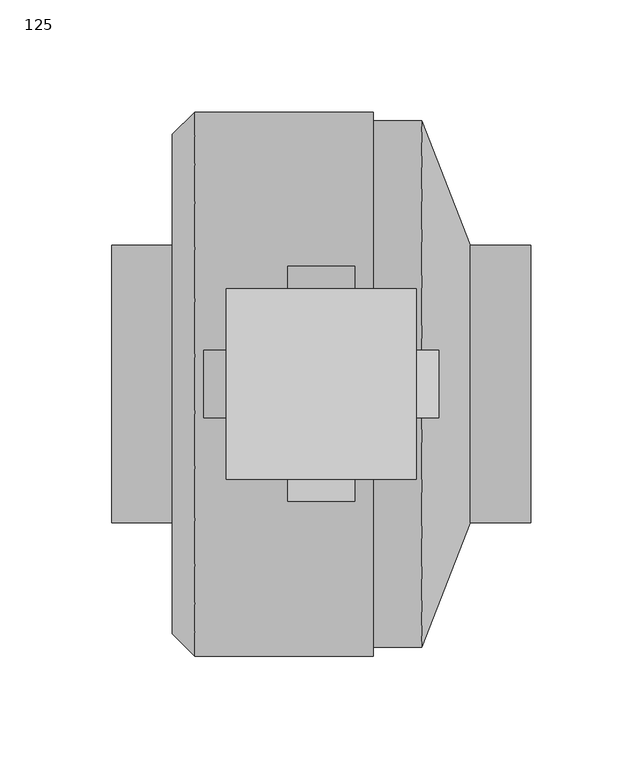
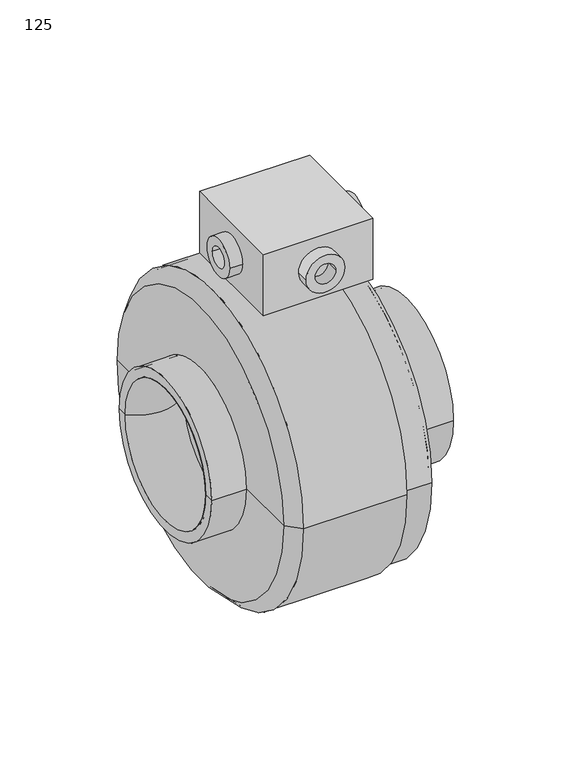
"""IFC4 building model written with IfcOpenShell, lengths in millimetres: proxy geometry, ВЕЗА_Канал-ВЕНТ : 125."""

from ifc_helpers import new_model, si_unit, point, frame, frame_2d, origin, place, context, project, spatial, polyline, circle_curve, ellipse_curve, trimmed, segment, composite_curve, outline, extrude, source, transform, mapped, element, save
from ifc_brep_helpers import plane_surface, cylinder_surface, revolved_surface, advanced_brep


def proxy_125_3bba99a2(model_context):
    return source(origin(), model_context, "Body", "SolidModel", [
        extrude(outline(composite_curve([segment(trimmed(circle_curve(frame_2d((0.0, 147.0)), 15.0), [point((-15.0, 147.0))], [point((15.0, 147.0))], False, "CARTESIAN"), True, "CONTINUOUS"), segment(trimmed(circle_curve(frame_2d((0.0, 147.0)), 15.0), [point((15.0, 147.0))], [point((-15.0, 147.0))], False, "CARTESIAN"), True, "CONTINUOUS")], self_intersect=False), holes=[composite_curve([segment(trimmed(circle_curve(frame_2d((0.0, 147.0)), 8.0), [point((-8.0, 147.0))], [point((8.0, 147.0))], True, "CARTESIAN"), True, "CONTINUOUS"), segment(trimmed(circle_curve(frame_2d((0.0, 147.0)), 8.0), [point((8.0, 147.0))], [point((-8.0, 147.0))], True, "CARTESIAN"), True, "CONTINUOUS")], self_intersect=False)]), frame((42.5, 0.0, 0.0), z_axis=(1.0, 0.0, 0.0), x_axis=(0.0, 1.0, 0.0)), (0.0, 0.0, 1.0), 10.0),
        extrude(outline(composite_curve([segment(trimmed(circle_curve(frame_2d((0.0, 147.0)), 15.0), [point((-15.0, 147.0))], [point((15.0, 147.0))], False, "CARTESIAN"), True, "CONTINUOUS"), segment(trimmed(circle_curve(frame_2d((0.0, 147.0)), 15.0), [point((15.0, 147.0))], [point((-15.0, 147.0))], False, "CARTESIAN"), True, "CONTINUOUS")], self_intersect=False), holes=[composite_curve([segment(trimmed(circle_curve(frame_2d((0.0, 147.0)), 8.0), [point((-8.0, 147.0))], [point((8.0, 147.0))], True, "CARTESIAN"), True, "CONTINUOUS"), segment(trimmed(circle_curve(frame_2d((0.0, 147.0)), 8.0), [point((8.0, 147.0))], [point((-8.0, 147.0))], True, "CARTESIAN"), True, "CONTINUOUS")], self_intersect=False)]), frame((-52.5, 0.0, 0.0), z_axis=(1.0, 0.0, 0.0), x_axis=(0.0, 1.0, 0.0)), (0.0, 0.0, 1.0), 10.0),
        extrude(outline(composite_curve([segment(trimmed(circle_curve(frame_2d((147.0, 0.0)), 15.0), [point((147.0, 15.0))], [point((147.0, -15.0))], False, "CARTESIAN"), True, "CONTINUOUS"), segment(trimmed(circle_curve(frame_2d((147.0, 0.0)), 15.0), [point((147.0, -15.0))], [point((147.0, 15.0))], False, "CARTESIAN"), True, "CONTINUOUS")], self_intersect=False), holes=[composite_curve([segment(trimmed(circle_curve(frame_2d((147.0, 0.0)), 8.0), [point((147.0, 8.0))], [point((147.0, -8.0))], True, "CARTESIAN"), True, "CONTINUOUS"), segment(trimmed(circle_curve(frame_2d((147.0, 0.0)), 8.0), [point((147.0, -8.0))], [point((147.0, 8.0))], True, "CARTESIAN"), True, "CONTINUOUS")], self_intersect=False)]), frame((0.0, -52.5, 0.0), z_axis=(0.0, 1.0, 0.0), x_axis=(0.0, 0.0, 1.0)), (0.0, 0.0, 1.0), 10.0),
        extrude(outline(composite_curve([segment(trimmed(circle_curve(frame_2d((147.0, 0.0)), 15.0), [point((147.0, 15.0))], [point((147.0, -15.0))], False, "CARTESIAN"), True, "CONTINUOUS"), segment(trimmed(circle_curve(frame_2d((147.0, 0.0)), 15.0), [point((147.0, -15.0))], [point((147.0, 15.0))], False, "CARTESIAN"), True, "CONTINUOUS")], self_intersect=False), holes=[composite_curve([segment(trimmed(circle_curve(frame_2d((147.0, 0.0)), 8.0), [point((147.0, 8.0))], [point((147.0, -8.0))], True, "CARTESIAN"), True, "CONTINUOUS"), segment(trimmed(circle_curve(frame_2d((147.0, 0.0)), 8.0), [point((147.0, -8.0))], [point((147.0, 8.0))], True, "CARTESIAN"), True, "CONTINUOUS")], self_intersect=False)]), frame((0.0, 42.5, 0.0), z_axis=(0.0, 1.0, 0.0), x_axis=(0.0, 0.0, 1.0)), (0.0, 0.0, 1.0), 10.0),
        extrude(outline(polyline([(-42.5, -42.5), (-42.5, 42.5), (42.5, 42.5), (42.5, -42.5), (-42.5, -42.5)])), frame((0.0, 0.0, 121.5), z_axis=(0.0, 0.0, 1.0), x_axis=(1.0, 0.0, 0.0)), (0.0, 0.0, 1.0), 50.0),
        advanced_brep(
        [(-93.5, -54.0, 0.0), (-93.5, 54.0, 0.0), (-92.0, 54.0, 0.0), (-92.0, -54.0, 0.0), (-48.5, -54.0, 0.0), (-48.5, 54.0, 0.0), (-50.0, -54.0, 0.0), (-50.0, 54.0, 0.0)],
        [
            (0, 1, circle_curve(frame((-93.5, 0.0, 0.0), z_axis=(1.0, 0.0, 0.0), x_axis=(0.0, 1.0, 0.0)), 54.0)),
            (1, 2),
            (2, 3, circle_curve(frame((-92.0, 0.0, 0.0), z_axis=(-1.0, 0.0, 0.0), x_axis=(0.0, 1.0, 0.0)), 54.0)),
            (3, 0),
            (1, 0, circle_curve(frame((-93.5, 0.0, 0.0), z_axis=(1.0, 0.0, 0.0), x_axis=(0.0, 1.0, 0.0)), 54.0)),
            (3, 2, circle_curve(frame((-92.0, 0.0, 0.0), z_axis=(-1.0, 0.0, 0.0), x_axis=(0.0, 1.0, 0.0)), 54.0)),
            (4, 5, circle_curve(frame((-48.5, 0.0, 0.0), z_axis=(1.0, 0.0, 0.0), x_axis=(0.0, 1.0, 0.0)), 54.0)),
            (5, 1, circle_curve(frame((-71.0, 77.6335583, 0.0), z_axis=(0.0, 0.0, -1.0), x_axis=(1.0, 0.0, 0.0)), 32.6311979)),
            (0, 4, circle_curve(frame((-71.0, -77.6335583, 0.0), z_axis=(0.0, 0.0, -1.0), x_axis=(1.0, 0.0, 0.0)), 32.6311979)),
            (5, 4, circle_curve(frame((-48.5, 0.0, 0.0), z_axis=(1.0, 0.0, 0.0), x_axis=(0.0, 1.0, 0.0)), 54.0)),
            (6, 7, circle_curve(frame((-50.0, 0.0, 0.0), z_axis=(1.0, 0.0, 0.0), x_axis=(0.0, 1.0, 0.0)), 54.0)),
            (7, 5),
            (4, 6),
            (7, 6, circle_curve(frame((-50.0, 0.0, 0.0), z_axis=(1.0, 0.0, 0.0), x_axis=(0.0, 1.0, 0.0)), 54.0)),
            (2, 7, circle_curve(frame((-71.0, 77.7023679, 0.0), z_axis=(0.0, 0.0, 1.0), x_axis=(1.0, 0.0, 0.0)), 31.667053)),
            (6, 3, circle_curve(frame((-71.0, -77.7023679, 0.0), z_axis=(0.0, 0.0, 1.0), x_axis=(1.0, 0.0, 0.0)), 31.667053)),
        ],
        [
            cylinder_surface(frame((-138.5, 0.0, 0.0), z_axis=(-1.0, 0.0, 0.0), x_axis=(0.0, 1.0, 0.0)), 54.0),
            revolved_surface(trimmed(ellipse_curve(frame((-71.0, 77.6335583, 0.0), z_axis=(0.0, 0.0, 1.0), x_axis=(1.0, 0.0, 0.0)), 32.6311979, 32.6311979), [point((-93.5, 54.0, 0.0))], [point((-48.5, 54.0, 0.0))], True, "CARTESIAN"), (-138.5, 0.0, 0.0), (-1.0, 0.0, 0.0)),
            revolved_surface(trimmed(ellipse_curve(frame((-71.0, 77.7023679, 0.0), z_axis=(0.0, 0.0, -1.0), x_axis=(1.0, 0.0, 0.0)), 31.667053, 31.667053), [point((-50.0, 54.0, 0.0))], [point((-92.0, 54.0, 0.0))], True, "CARTESIAN"), (-138.5, 0.0, 0.0), (-1.0, 0.0, 0.0)),
        ],
        [
            (0, [[1, 2, 3, 4]]),
            (0, [[5, -4, 6, -2]]),
            (1, [[7, 8, -1, 9]]),
            (1, [[10, -9, -5, -8]]),
            (0, [[11, 12, -7, 13]]),
            (0, [[14, -13, -10, -12]]),
            (2, [[-3, 15, -11, 16]]),
            (2, [[-6, -16, -14, -15]]),
        ],
    ),
        advanced_brep(
        [(-92.0, -60.5, 0.0), (-92.0, 60.5, 0.0), (-92.0, 54.0, 0.0), (-92.0, -54.0, 0.0), (21.6666667, -120.0, 0.0), (21.6666667, 120.0, 0.0), (-56.5, 120.0, 0.0), (-56.5, -120.0, 0.0), (21.6666667, -116.0, 0.0), (21.6666667, 116.0, 0.0), (43.3333333, -116.0, 0.0), (43.3333333, 116.0, 0.0), (65.0, -60.5, 0.0), (65.0, 60.5, 0.0), (93.5, -60.5, 0.0), (93.5, 60.5, 0.0), (93.5, -62.0, 0.0), (93.5, 62.0, 0.0), (66.5, -62.0, 0.0), (66.5, 62.0, 0.0), (44.8333333, -117.5, 0.0), (44.8333333, 117.5, 0.0), (23.1666667, -117.5, 0.0), (23.1666667, 117.5, 0.0), (23.1666667, -121.5, 0.0), (23.1666667, 121.5, 0.0), (-56.5, -121.5, 0.0), (-56.5, 121.5, 0.0), (-66.5, -62.0, 0.0), (-66.5, 62.0, 0.0), (-66.5, 111.5, 0.0), (-66.5, -111.5, 0.0), (-93.5, -62.0, 0.0), (-93.5, 62.0, 0.0), (-93.5, -54.0, 0.0), (-93.5, 54.0, 0.0), (-65.0, -60.5, 0.0), (-65.0, 60.5, 0.0), (-65.0, -111.5, 0.0), (-65.0, 111.5, 0.0)],
        [
            (0, 1, circle_curve(frame((-92.0, 0.0, 0.0), z_axis=(1.0, 0.0, 0.0), x_axis=(0.0, 1.0, 0.0)), 60.5)),
            (1, 2),
            (2, 3, circle_curve(frame((-92.0, 0.0, 0.0), z_axis=(-1.0, 0.0, 0.0), x_axis=(0.0, 1.0, 0.0)), 54.0)),
            (3, 0),
            (1, 0, circle_curve(frame((-92.0, 0.0, 0.0), z_axis=(1.0, 0.0, 0.0), x_axis=(0.0, 1.0, 0.0)), 60.5)),
            (3, 2, circle_curve(frame((-92.0, 0.0, 0.0), z_axis=(-1.0, 0.0, 0.0), x_axis=(0.0, 1.0, 0.0)), 54.0)),
            (4, 5, circle_curve(frame((21.6666667, 0.0, 0.0), z_axis=(1.0, 0.0, 0.0), x_axis=(0.0, 1.0, 0.0)), 120.0)),
            (5, 6),
            (6, 7, circle_curve(frame((-56.5, 0.0, 0.0), z_axis=(-1.0, 0.0, 0.0), x_axis=(0.0, 1.0, 0.0)), 120.0)),
            (7, 4),
            (5, 4, circle_curve(frame((21.6666667, 0.0, 0.0), z_axis=(1.0, 0.0, 0.0), x_axis=(0.0, 1.0, 0.0)), 120.0)),
            (7, 6, circle_curve(frame((-56.5, 0.0, 0.0), z_axis=(-1.0, 0.0, 0.0), x_axis=(0.0, 1.0, 0.0)), 120.0)),
            (8, 9, circle_curve(frame((21.6666667, 0.0, 0.0), z_axis=(1.0, 0.0, 0.0), x_axis=(0.0, 1.0, 0.0)), 116.0)),
            (9, 5),
            (4, 8),
            (9, 8, circle_curve(frame((21.6666667, 0.0, 0.0), z_axis=(1.0, 0.0, 0.0), x_axis=(0.0, 1.0, 0.0)), 116.0)),
            (10, 11, circle_curve(frame((43.3333333, 0.0, 0.0), z_axis=(1.0, 0.0, 0.0), x_axis=(0.0, 1.0, 0.0)), 116.0)),
            (11, 9),
            (8, 10),
            (11, 10, circle_curve(frame((43.3333333, 0.0, 0.0), z_axis=(1.0, 0.0, 0.0), x_axis=(0.0, 1.0, 0.0)), 116.0)),
            (12, 13, circle_curve(frame((65.0, 0.0, 0.0), z_axis=(1.0, 0.0, 0.0), x_axis=(0.0, 1.0, 0.0)), 60.5)),
            (13, 11),
            (10, 12),
            (13, 12, circle_curve(frame((65.0, 0.0, 0.0), z_axis=(1.0, 0.0, 0.0), x_axis=(0.0, 1.0, 0.0)), 60.5)),
            (14, 15, circle_curve(frame((93.5, 0.0, 0.0), z_axis=(1.0, 0.0, 0.0), x_axis=(0.0, 1.0, 0.0)), 60.5)),
            (15, 13),
            (12, 14),
            (15, 14, circle_curve(frame((93.5, 0.0, 0.0), z_axis=(1.0, 0.0, 0.0), x_axis=(0.0, 1.0, 0.0)), 60.5)),
            (16, 17, circle_curve(frame((93.5, 0.0, 0.0), z_axis=(1.0, 0.0, 0.0), x_axis=(0.0, 1.0, 0.0)), 62.0)),
            (17, 15),
            (14, 16),
            (17, 16, circle_curve(frame((93.5, 0.0, 0.0), z_axis=(1.0, 0.0, 0.0), x_axis=(0.0, 1.0, 0.0)), 62.0)),
            (18, 19, circle_curve(frame((66.5, 0.0, 0.0), z_axis=(1.0, 0.0, 0.0), x_axis=(0.0, 1.0, 0.0)), 62.0)),
            (19, 17),
            (16, 18),
            (19, 18, circle_curve(frame((66.5, 0.0, 0.0), z_axis=(1.0, 0.0, 0.0), x_axis=(0.0, 1.0, 0.0)), 62.0)),
            (20, 21, circle_curve(frame((44.8333333, 0.0, 0.0), z_axis=(1.0, 0.0, 0.0), x_axis=(0.0, 1.0, 0.0)), 117.5)),
            (21, 19),
            (18, 20),
            (21, 20, circle_curve(frame((44.8333333, 0.0, 0.0), z_axis=(1.0, 0.0, 0.0), x_axis=(0.0, 1.0, 0.0)), 117.5)),
            (22, 23, circle_curve(frame((23.1666667, 0.0, 0.0), z_axis=(1.0, 0.0, 0.0), x_axis=(0.0, 1.0, 0.0)), 117.5)),
            (23, 21),
            (20, 22),
            (23, 22, circle_curve(frame((23.1666667, 0.0, 0.0), z_axis=(1.0, 0.0, 0.0), x_axis=(0.0, 1.0, 0.0)), 117.5)),
            (24, 25, circle_curve(frame((23.1666667, 0.0, 0.0), z_axis=(1.0, 0.0, 0.0), x_axis=(0.0, 1.0, 0.0)), 121.5)),
            (25, 23),
            (22, 24),
            (25, 24, circle_curve(frame((23.1666667, 0.0, 0.0), z_axis=(1.0, 0.0, 0.0), x_axis=(0.0, 1.0, 0.0)), 121.5)),
            (26, 27, circle_curve(frame((-56.5, 0.0, 0.0), z_axis=(1.0, 0.0, 0.0), x_axis=(0.0, 1.0, 0.0)), 121.5)),
            (27, 25),
            (24, 26),
            (27, 26, circle_curve(frame((-56.5, 0.0, 0.0), z_axis=(1.0, 0.0, 0.0), x_axis=(0.0, 1.0, 0.0)), 121.5)),
            (28, 29, circle_curve(frame((-66.5, 0.0, 0.0), z_axis=(1.0, 0.0, 0.0), x_axis=(0.0, 1.0, 0.0)), 62.0)),
            (29, 30),
            (30, 31, circle_curve(frame((-66.5, 0.0, 0.0), z_axis=(-1.0, 0.0, 0.0), x_axis=(0.0, 1.0, 0.0)), 111.5)),
            (31, 28),
            (29, 28, circle_curve(frame((-66.5, 0.0, 0.0), z_axis=(1.0, 0.0, 0.0), x_axis=(0.0, 1.0, 0.0)), 62.0)),
            (31, 30, circle_curve(frame((-66.5, 0.0, 0.0), z_axis=(-1.0, 0.0, 0.0), x_axis=(0.0, 1.0, 0.0)), 111.5)),
            (32, 33, circle_curve(frame((-93.5, 0.0, 0.0), z_axis=(1.0, 0.0, 0.0), x_axis=(0.0, 1.0, 0.0)), 62.0)),
            (33, 29),
            (28, 32),
            (33, 32, circle_curve(frame((-93.5, 0.0, 0.0), z_axis=(1.0, 0.0, 0.0), x_axis=(0.0, 1.0, 0.0)), 62.0)),
            (34, 35, circle_curve(frame((-93.5, 0.0, 0.0), z_axis=(1.0, 0.0, 0.0), x_axis=(0.0, 1.0, 0.0)), 54.0)),
            (35, 33),
            (32, 34),
            (35, 34, circle_curve(frame((-93.5, 0.0, 0.0), z_axis=(1.0, 0.0, 0.0), x_axis=(0.0, 1.0, 0.0)), 54.0)),
            (2, 35),
            (34, 3),
            (36, 37, circle_curve(frame((-65.0, 0.0, 0.0), z_axis=(1.0, 0.0, 0.0), x_axis=(0.0, 1.0, 0.0)), 60.5)),
            (37, 1),
            (0, 36),
            (37, 36, circle_curve(frame((-65.0, 0.0, 0.0), z_axis=(1.0, 0.0, 0.0), x_axis=(0.0, 1.0, 0.0)), 60.5)),
            (38, 39, circle_curve(frame((-65.0, 0.0, 0.0), z_axis=(1.0, 0.0, 0.0), x_axis=(0.0, 1.0, 0.0)), 111.5)),
            (39, 37),
            (36, 38),
            (39, 38, circle_curve(frame((-65.0, 0.0, 0.0), z_axis=(1.0, 0.0, 0.0), x_axis=(0.0, 1.0, 0.0)), 111.5)),
            (6, 39),
            (38, 7),
            (30, 27),
            (26, 31),
        ],
        [
            plane_surface(frame((-92.0, 0.0, 0.0), z_axis=(1.0, 0.0, 0.0), x_axis=(0.0, 1.0, 0.0))),
            revolved_surface(polyline([(-56.5, 120.0, 0.0), (21.666666700000007, 120.0, 0.0)]), (-163.5, 0.0, 0.0), (-1.0, 0.0, 0.0)),
            plane_surface(frame((21.6666667, 0.0, 0.0), z_axis=(-1.0, 0.0, 0.0), x_axis=(0.0, 1.0, 0.0))),
            revolved_surface(polyline([(21.666666700000007, 116.0, 0.0), (43.33333329999999, 116.0, 0.0)]), (-163.5, 0.0, 0.0), (-1.0, 0.0, 0.0)),
            revolved_surface(polyline([(43.3333333, 116.0, 0.0), (65.0, 60.5, 0.0)]), (-163.5, 0.0, 0.0), (-1.0, 0.0, 0.0)),
            revolved_surface(polyline([(65.0, 60.5, 0.0), (93.5, 60.5, 0.0)]), (-163.5, 0.0, 0.0), (-1.0, 0.0, 0.0)),
            plane_surface(frame((93.5, 0.0, 0.0), z_axis=(1.0, 0.0, 0.0), x_axis=(0.0, 1.0, 0.0))),
            cylinder_surface(frame((-163.5, 0.0, 0.0), z_axis=(-1.0, 0.0, 0.0), x_axis=(0.0, 1.0, 0.0)), 62.0),
            revolved_surface(polyline([(66.5, 62.0, 0.0), (44.8333333, 117.5, 0.0)]), (-163.5, 0.0, 0.0), (-1.0, 0.0, 0.0)),
            cylinder_surface(frame((-163.5, 0.0, 0.0), z_axis=(-1.0, 0.0, 0.0), x_axis=(0.0, 1.0, 0.0)), 117.5),
            plane_surface(frame((23.1666667, 0.0, 0.0), z_axis=(1.0, 0.0, 0.0), x_axis=(0.0, 1.0, 0.0))),
            cylinder_surface(frame((-163.5, 0.0, 0.0), z_axis=(-1.0, 0.0, 0.0), x_axis=(0.0, 1.0, 0.0)), 121.5),
            plane_surface(frame((-66.5, 0.0, 0.0), z_axis=(-1.0, 0.0, 0.0), x_axis=(0.0, 1.0, 0.0))),
            plane_surface(frame((-93.5, 0.0, 0.0), z_axis=(-1.0, 0.0, 0.0), x_axis=(0.0, 1.0, 0.0))),
            revolved_surface(polyline([(-93.5, 54.0, 0.0), (-92.0, 54.0, 0.0)]), (-163.5, 0.0, 0.0), (-1.0, 0.0, 0.0)),
            revolved_surface(polyline([(-92.0, 60.5, 0.0), (-65.0, 60.5, 0.0)]), (-163.5, 0.0, 0.0), (-1.0, 0.0, 0.0)),
            plane_surface(frame((-65.0, 0.0, 0.0), z_axis=(1.0, 0.0, 0.0), x_axis=(0.0, 1.0, 0.0))),
            revolved_surface(polyline([(-65.0, 111.5, 0.0), (-56.5, 120.0, 0.0)]), (-163.5, 0.0, 0.0), (-1.0, 0.0, 0.0)),
            revolved_surface(polyline([(-56.5, 121.5, 0.0), (-66.5, 111.5, 0.0)]), (-163.5, 0.0, 0.0), (-1.0, 0.0, 0.0)),
        ],
        [
            (0, [[1, 2, 3, 4]]),
            (0, [[5, -4, 6, -2]]),
            (1, [[7, 8, 9, 10]]),
            (1, [[11, -10, 12, -8]]),
            (2, [[13, 14, -7, 15]]),
            (2, [[16, -15, -11, -14]]),
            (3, [[17, 18, -13, 19]]),
            (3, [[20, -19, -16, -18]]),
            (4, [[21, 22, -17, 23]]),
            (4, [[24, -23, -20, -22]]),
            (5, [[25, 26, -21, 27]]),
            (5, [[28, -27, -24, -26]]),
            (6, [[29, 30, -25, 31]]),
            (6, [[32, -31, -28, -30]]),
            (7, [[33, 34, -29, 35]]),
            (7, [[36, -35, -32, -34]]),
            (8, [[37, 38, -33, 39]]),
            (8, [[40, -39, -36, -38]]),
            (9, [[41, 42, -37, 43]]),
            (9, [[44, -43, -40, -42]]),
            (10, [[45, 46, -41, 47]]),
            (10, [[48, -47, -44, -46]]),
            (11, [[49, 50, -45, 51]]),
            (11, [[52, -51, -48, -50]]),
            (12, [[53, 54, 55, 56]]),
            (12, [[57, -56, 58, -54]]),
            (7, [[59, 60, -53, 61]]),
            (7, [[62, -61, -57, -60]]),
            (13, [[63, 64, -59, 65]]),
            (13, [[66, -65, -62, -64]]),
            (14, [[-3, 67, -63, 68]]),
            (14, [[-6, -68, -66, -67]]),
            (15, [[69, 70, -1, 71]]),
            (15, [[72, -71, -5, -70]]),
            (16, [[73, 74, -69, 75]]),
            (16, [[76, -75, -72, -74]]),
            (17, [[-9, 77, -73, 78]]),
            (17, [[-12, -78, -76, -77]]),
            (18, [[-55, 79, -49, 80]]),
            (18, [[-58, -80, -52, -79]]),
        ],
    ),
        advanced_brep(
        [(0.0, -91.75, 0.0), (0.0, 91.75, 0.0), (0.0, 0.0, 0.0), (-48.5, -91.75, 0.0), (-48.5, 91.75, 0.0), (-48.5, 0.0, 0.0)],
        [
            (0, 1, circle_curve(frame((0.0, 0.0, 0.0), z_axis=(1.0, 0.0, 0.0), x_axis=(0.0, 1.0, 0.0)), 91.75)),
            (1, 2),
            (2, 0),
            (1, 0, circle_curve(frame((0.0, 0.0, 0.0), z_axis=(1.0, 0.0, 0.0), x_axis=(0.0, 1.0, 0.0)), 91.75)),
            (3, 4, circle_curve(frame((-48.5, 0.0, 0.0), z_axis=(1.0, 0.0, 0.0), x_axis=(0.0, 1.0, 0.0)), 91.75)),
            (4, 1),
            (0, 3),
            (4, 3, circle_curve(frame((-48.5, 0.0, 0.0), z_axis=(1.0, 0.0, 0.0), x_axis=(0.0, 1.0, 0.0)), 91.75)),
            (5, 4),
            (3, 5),
        ],
        [
            plane_surface(frame((0.0, 0.0, 0.0), z_axis=(1.0, 0.0, 0.0), x_axis=(0.0, 1.0, 0.0))),
            cylinder_surface(frame((-183.5, 0.0, 0.0), z_axis=(-1.0, 0.0, 0.0), x_axis=(0.0, 1.0, 0.0)), 91.75),
            plane_surface(frame((-48.5, 0.0, 0.0), z_axis=(-1.0, 0.0, 0.0), x_axis=(0.0, 1.0, 0.0))),
        ],
        [
            (0, [[1, 2, 3]]),
            (0, [[4, -3, -2]]),
            (1, [[5, 6, -1, 7]]),
            (1, [[8, -7, -4, -6]]),
            (2, [[9, -5, 10]]),
            (2, [[-10, -8, -9]]),
        ],
    ),
    ])


if __name__ == "__main__":
    model = new_model("IFC4")
    model_context = context("Model", 3, world=origin())
    ifc_project = project(units=[si_unit("LENGTHUNIT", "METRE", prefix="MILLI")], contexts=[model_context])
    site = spatial("IfcSite", under=ifc_project)
    building = spatial("IfcBuilding", under=site)
    placement = place(None, origin())
    proxy_125_shape = proxy_125_3bba99a2(model_context)
    element("IfcBuildingElementProxy", 1, Name="ВЕЗА_Канал-ВЕНТ : 125", ObjectType="ВЕЗА_Канал-ВЕНТ : 125", at=placement, inside=building, context=model_context, shape_type="MappedRepresentation", body=[
        mapped(proxy_125_shape, transform((0.0, 0.0, 0.0), x_axis=(1.0, 0.0, 0.0), y_axis=(0.0, 1.0, 0.0), z_axis=(0.0, 0.0, 1.0))),
    ])
    save(model, "model.ifc")

# Revit data of these elements
# Type "ВЕЗА_Канал-ВЕНТ : 125"
#   ВЕЗА_Классификатор = "11031"
#   ВЕЗА_Контакты = "bim@veza.ru"
#   URL = "http://www.veza.ru/docs/sistemy-kanalnoy-ventilyatsii-kanal/"
#   Таблица = "kanal-vent"
#   ADSK_Примечание = ""
#   ADSK_Позиция на схеме = ""
#   ADSK_Позиция = ""
#   ADSK_Наименование краткое = "Канал-ВЕНТ"
#   ADSK_Наименование = "Вентилятор канальный для круглых каналов"
#   ADSK_Марка = "Канал-ВЕНТ-125"
#   ADSK_Комплект [instance default] = ""
#   ADSK_Код изделия = ""
#   ADSK_Завод-изготовитель = "ООО \"Веза\", Россия, Москва, ИНН 505001001, info@veza.ru"
#   ADSK_Единица измерения = "компл."
#   ADSK_Дата изменения = "10.03.2020"
#   ADSK_Группирование = ""
#   ADSK_Версия семейства = "Версия 4"
#   ADSK_Версия Revit = "Revit 2017"
#   Угол поворота УГО 3D [instance default] = 45°
#   L [instance default] = 187 mm
#   h [instance default] = 27 mm
#   D [instance default] = 243 mm
#   ADSK_Ток [instance default] = 0.29 A
#   ADSK_Расход воздуха [instance default] = 561.6 m³/h
#   ADSK_Размер_Диаметр [instance default] = 124 mm
#   ADSK_Полная мощность [instance default] = 65 VA
#   ADSK_Номинальная мощность [instance default] = 65 W
#   ADSK_Напряжение = 230 V
#   ADSK_Масса [instance default] = 3.3
#   ADSK_Коэффициент мощности = 1
#   ADSK_Количество = 1
#   Масштаб УГО [instance default] = 100
#   ВЕЗА_Типоразмер = 125
#   ВЕЗА_Число полюсов = 2
#   ADSK_Частота вращения двигателя [instance default] = 2400
#   ADSK_Количество фаз = 1
#   Материал = ВЕЗА_Оцинкованная сталь
#   Default Elevation = 0
#   Description = (empty or 0)
#   Type Image = (empty or 0)
#   Manufacturer = ""
# Element 1 (IfcBuildingElementProxy, "ВЕЗА_Канал-ВЕНТ : 125")
#   Materials on its faces: "ВЕЗА_Оцинкованная сталь", "Пластмасса коробки"
# Materials
#   "ВЕЗА_Оцинкованная сталь": class "Типовые", colour RGB 120 120 120, transparency 0, Cost = 0
#   "Пластмасса коробки": class "Типовые", colour RGB 120 120 120, transparency 0, Cost = 0
